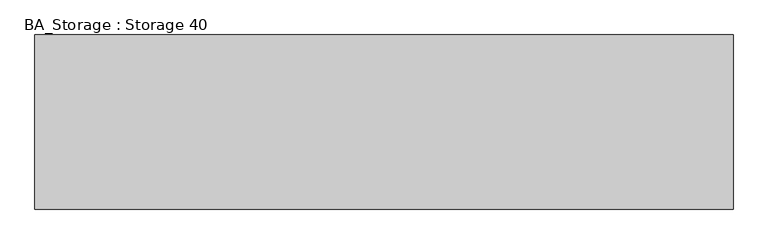
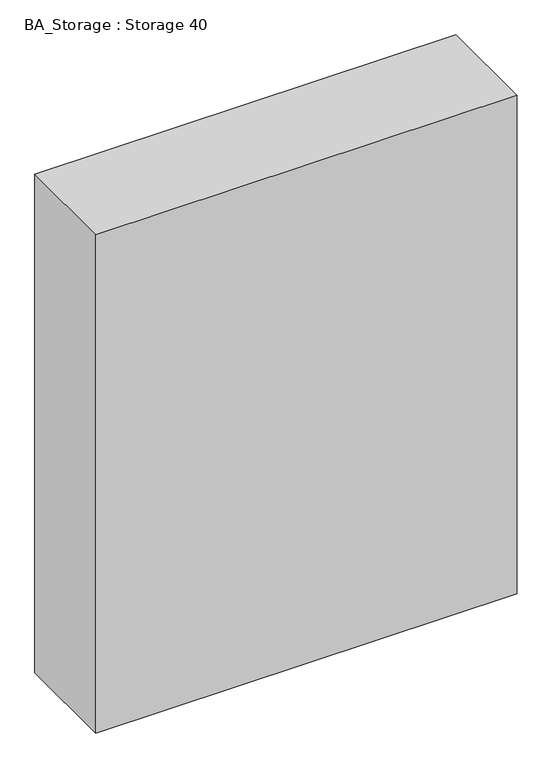
"""IFC4 building model written with IfcOpenShell, lengths in millimetres: furniture geometry, BA_Storage : Storage 40."""

from ifc_helpers import new_model, si_unit, origin, origin_with_axes, place, context, project, spatial, polyline, outline, extrude, source, transform, mapped, element, save


def ba_storage_storage_40_a302475e(model_context):
    return source(origin(), model_context, "Body", "SweptSolid", [
        extrude(outline(polyline([(1600.0, 0.0), (0.0, 0.0), (0.0, 400.0), (1600.0, 400.0), (1600.0, 0.0)])), origin_with_axes(), (0.0, 0.0, 1.0), 2000.0),
    ])


if __name__ == "__main__":
    model = new_model("IFC4")
    model_context = context("Model", 3, world=origin())
    ifc_project = project(units=[si_unit("LENGTHUNIT", "METRE", prefix="MILLI")], contexts=[model_context])
    site = spatial("IfcSite", under=ifc_project)
    building = spatial("IfcBuilding", under=site)
    placement = place(None, origin())
    ba_storage_storage_40_shape = ba_storage_storage_40_a302475e(model_context)
    element("IfcFurniture", 1, ObjectType="BA_Storage : Storage 40", at=placement, inside=building, context=model_context, shape_type="MappedRepresentation", body=[
        mapped(ba_storage_storage_40_shape, transform((0.0, 0.0, 0.0), x_axis=(1.0, 0.0, 0.0), y_axis=(0.0, 1.0, 0.0), z_axis=(0.0, 0.0, 1.0))),
    ])
    save(model, "model.ifc")

# Revit data of these elements
# Type "BA_Storage : Storage 40"
#   built-in parameter 1001306 [instance default] = 4.85564 (stored number, unit not read)
#   Height [instance default] = 2000 mm
#   depth = 400 mm
#   Default Elevation = 0
# Element 1 (IfcFurniture, "BA_Storage : Storage 40")
#   built-in parameter 1001306 = 5.24934 (stored number, unit not read)
#   Materials on its faces: "Default"
# Materials
#   "Default": class "Generic", colour RGB 255 255 255, transparency 0, Cost = 0
